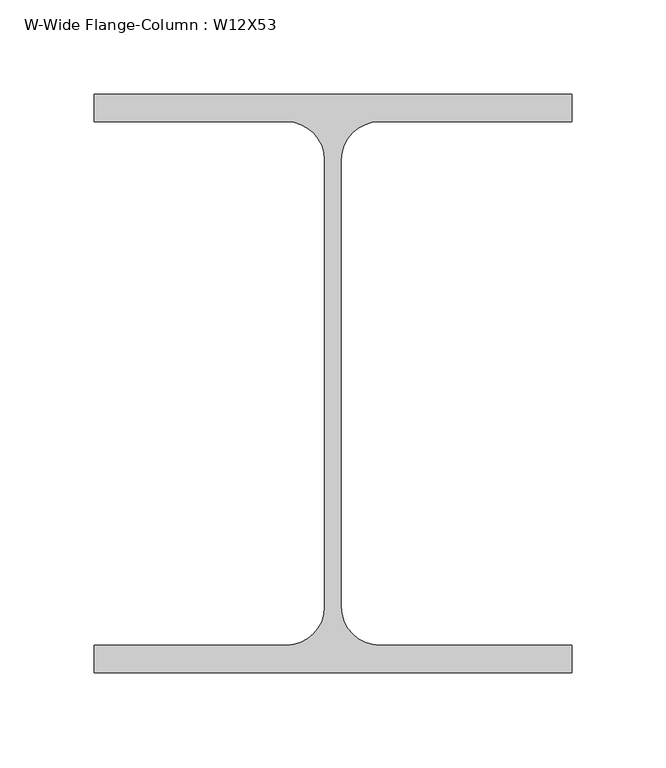
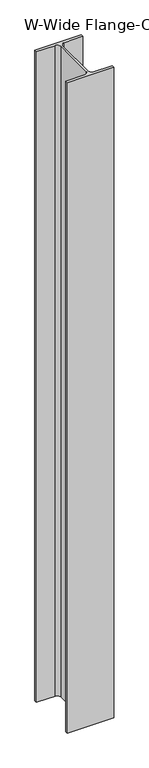
"""IFC4 building model written with IfcOpenShell, lengths in millimetres: column geometry, W-Wide Flange-Column : W12X53."""

from ifc_helpers import new_model, si_unit, point, frame, frame_2d, origin, place, context, project, spatial, polyline, circle_curve, trimmed, segment, composite_curve, outline, extrude, source, transform, mapped, element, save


def w_wide_flange_column_w12x53_e48874d2(model_context):
    return source(origin(), model_context, "Body", "SweptSolid", [
        extrude(outline(composite_curve([segment(polyline([(127.0, 153.67), (127.0, 139.065), (24.7015, 139.065)]), True, "CONTINUOUS"), segment(trimmed(circle_curve(frame_2d((24.7015, 118.745)), 20.32), [point((24.7015, 139.065))], [point((4.3815, 118.745))], True, "CARTESIAN"), True, "CONTINUOUS"), segment(polyline([(4.3815, 118.745), (4.3815, -118.745)]), True, "CONTINUOUS"), segment(trimmed(circle_curve(frame_2d((24.7015, -118.745)), 20.32), [point((4.3815, -118.745))], [point((24.7015, -139.065))], True, "CARTESIAN"), True, "CONTINUOUS"), segment(polyline([(24.7015, -139.065), (127.0, -139.065), (127.0, -153.67), (-127.0, -153.67), (-127.0, -139.065), (-24.7015, -139.065)]), True, "CONTINUOUS"), segment(trimmed(circle_curve(frame_2d((-24.7015, -118.745)), 20.32), [point((-24.7015, -139.065))], [point((-4.3815, -118.745))], True, "CARTESIAN"), True, "CONTINUOUS"), segment(polyline([(-4.3815, -118.745), (-4.3815, 118.745)]), True, "CONTINUOUS"), segment(trimmed(circle_curve(frame_2d((-24.7015, 118.745)), 20.32), [point((-4.3815, 118.745))], [point((-24.7015, 139.065))], True, "CARTESIAN"), True, "CONTINUOUS"), segment(polyline([(-24.7015, 139.065), (-127.0, 139.065), (-127.0, 153.67), (127.0, 153.67)]), True, "CONTINUOUS")], self_intersect=False)), frame((0.0, 0.0, 8655.05), z_axis=(0.0, 0.0, 1.0), x_axis=(1.0, 0.0, 0.0)), (0.0, 0.0, 1.0), 3752.85),
    ])


if __name__ == "__main__":
    model = new_model("IFC4")
    model_context = context("Model", 3, world=origin())
    ifc_project = project(units=[si_unit("LENGTHUNIT", "METRE", prefix="MILLI")], contexts=[model_context])
    site = spatial("IfcSite", under=ifc_project)
    building = spatial("IfcBuilding", under=site)
    placement = place(None, origin())
    w_wide_flange_column_w12x53_shape = w_wide_flange_column_w12x53_e48874d2(model_context)
    element("IfcColumn", 1, ObjectType="W-Wide Flange-Column : W12X53", at=placement, inside=building, context=model_context, shape_type="MappedRepresentation", body=[
        mapped(w_wide_flange_column_w12x53_shape, transform((0.0, 0.0, 0.0), x_axis=(1.0, 0.0, 0.0), y_axis=(0.0, 1.0, 0.0), z_axis=(0.0, 0.0, 1.0))),
    ])
    save(model, "model.ifc")

# Revit data of these elements
# Type "W-Wide Flange-Column : W12X53"
#   Assembly Code = "B10"
#   W = 53
#   bf = 0' - 10"
#   d = 1' - 0.1"
#   k = 0' - 1 3/8"
#   kr = 0' - 0.8"
#   tf = 0' - 0.575"
#   tw = 0' - 0.345"
#   A = 0.108333 SF
#   Structural Material [instance default] = Steel ASTM A992
# Element 1 (IfcColumn, "W-Wide Flange-Column : W12X53")
#   Materials on its faces: "Steel ASTM A992"
# Materials
#   "Steel ASTM A992": class "Metal", colour RGB 199 199 199, transparency 0, Description = "Structural steel 50ksi", Cost = 0
